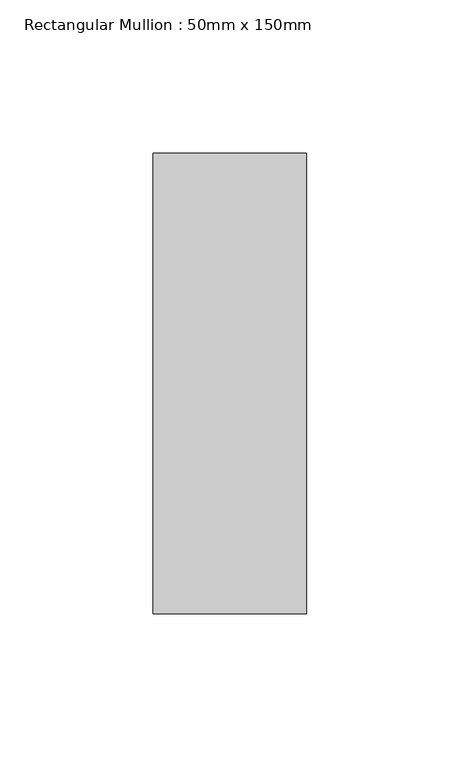
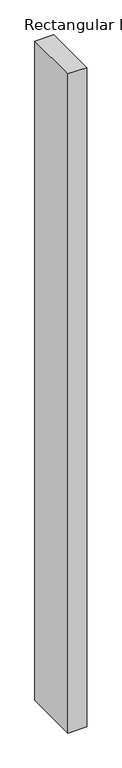
"""IFC4 building model written with IfcOpenShell, lengths in millimetres: member geometry, Rectangular Mullion : 50mm x 150mm."""

import ifcopenshell
import ifcopenshell.guid

model = None  # the IFC model being written
_history = None  # IfcOwnerHistory: only IFC2X3 demands one
_inside = {}  # id of a spatial element -> (the spatial element, [elements in it])
_under = {}  # id of a project, library or spatial element -> (it, [spatial elements below it])
_declared = {}  # id of a project -> (the project, [libraries it declares])
_typed = {}  # id of a type object -> (the type object, [elements of that type])
_made_of = {}  # id of a material, layer set ... -> (it, [elements and type objects made of it])


def new_model(schema):
    """Start an empty IFC model of exactly this schema.

    Asked for "IFC4X3", IfcOpenShell would pick the latest addendum, in which some entities
    have other attributes; the version numbers below select the first issue.
    IFC2X3 requires an IfcOwnerHistory on every rooted entity: one is made here for all.
    """
    global model, _history
    if schema == "IFC4X3":
        model = ifcopenshell.file(schema_version=(4, 3, 0, 0))
    else:
        model = ifcopenshell.file(schema=schema)
    _inside.clear()
    _under.clear()
    _declared.clear()
    _typed.clear()
    _made_of.clear()
    _history = None
    if model.schema == "IFC2X3":
        org = make("IfcOrganization", Name="unknown")
        user = make(
            "IfcPersonAndOrganization",
            ThePerson=make("IfcPerson", FamilyName="unknown"),
            TheOrganization=org,
        )
        app = make(
            "IfcApplication",
            ApplicationDeveloper=org,
            Version="unknown",
            ApplicationFullName="unknown",
            ApplicationIdentifier="unknown",
        )
        _history = make(
            "IfcOwnerHistory",
            OwningUser=user,
            OwningApplication=app,
            ChangeAction="ADDED",
            CreationDate=0,
        )
    return model


def make(cls, **values):
    """One entity of the class cls with the attributes given. An attribute that is None is left unset."""
    return model.create_entity(
        cls, **{name: value for name, value in values.items() if value is not None}
    )


def rooted(cls, **values):
    """An entity with a GlobalId (a new one), such as an element, a storey or a relation."""
    return make(cls, GlobalId=ifcopenshell.guid.new(), OwnerHistory=_history, **values)


def si_unit(unit_type, name, prefix=None):
    """IfcSIUnit, for example si_unit("LENGTHUNIT", "METRE", prefix="MILLI")."""
    return make("IfcSIUnit", UnitType=unit_type, Prefix=prefix, Name=name)


def assignment(units):
    """IfcUnitAssignment: the units of a project."""
    return None if units is None else make("IfcUnitAssignment", Units=units)


def point(xyz):
    """IfcCartesianPoint."""
    return None if xyz is None else make("IfcCartesianPoint", Coordinates=xyz)


def direction(xyz):
    """IfcDirection."""
    return None if xyz is None else make("IfcDirection", DirectionRatios=xyz)


def frame(location, z_axis=None, x_axis=None):
    """IfcAxis2Placement3D, a coordinate frame: its origin and axes. An axis left out is left unset."""
    return make(
        "IfcAxis2Placement3D",
        Location=point(location),
        Axis=direction(z_axis),
        RefDirection=direction(x_axis),
    )


def origin():
    """The frame at (0, 0, 0) with its axes left unset."""
    return frame((0.0, 0.0, 0.0))


def place(relative_to, where):
    """IfcLocalPlacement: puts the frame where relative to a parent placement (None: the world)."""
    return make(
        "IfcLocalPlacement", PlacementRelTo=relative_to, RelativePlacement=where
    )


def context(
    kind, dimensions, precision=None, world=None, true_north=None, identifier=None
):
    """IfcGeometricRepresentationContext, for example the 3D "Model" context."""
    return make(
        "IfcGeometricRepresentationContext",
        ContextIdentifier=identifier,
        ContextType=kind,
        CoordinateSpaceDimension=dimensions,
        Precision=precision,
        WorldCoordinateSystem=world,
        TrueNorth=true_north,
    )


def project(units=None, contexts=None):
    """IfcProject with its units and contexts."""
    return rooted(
        "IfcProject",
        Name="project",
        RepresentationContexts=contexts,
        UnitsInContext=assignment(units),
    )


def spatial(cls, under=None, at=None, **own):
    """A site, building, storey or space (cls), placed at a placement, below another one or the project."""
    s = rooted(cls, ObjectPlacement=at, **own)
    if under is not None:
        _under.setdefault(under.id(), (under, []))[1].append(s)
    return s


def polyline(points):
    """IfcPolyline through the points."""
    return make("IfcPolyline", Points=[point(p) for p in points])


def outline(outer, holes=None, kind="AREA"):
    """IfcArbitraryClosedProfileDef: a profile drawn as a closed curve; with holes, ...WithVoids."""
    if holes is None:
        return make("IfcArbitraryClosedProfileDef", ProfileType=kind, OuterCurve=outer)
    return make(
        "IfcArbitraryProfileDefWithVoids",
        ProfileType=kind,
        OuterCurve=outer,
        InnerCurves=holes,
    )


def extrude(swept, where, along, depth):
    """IfcExtrudedAreaSolid: the profile swept, set in the frame where, extruded along a direction by depth."""
    return make(
        "IfcExtrudedAreaSolid",
        SweptArea=swept,
        Position=where,
        ExtrudedDirection=direction(along),
        Depth=depth,
    )


def shape(context_of_items, identifier, shape_type, items):
    """IfcShapeRepresentation: the items that make up one representation, for example the "Body"."""
    return make(
        "IfcShapeRepresentation",
        ContextOfItems=context_of_items,
        RepresentationIdentifier=identifier,
        RepresentationType=shape_type,
        Items=items,
    )


def source(mapping_origin, context_of_items, identifier, shape_type, items):
    """IfcRepresentationMap: a shape defined once, which mapped items show again and again."""
    return make(
        "IfcRepresentationMap",
        MappingOrigin=mapping_origin,
        MappedRepresentation=shape(context_of_items, identifier, shape_type, items),
    )


def transform(
    local_origin,
    x_axis=None,
    y_axis=None,
    z_axis=None,
    scale=None,
    scale2=None,
    scale3=None,
    uniform=True,
):
    """IfcCartesianTransformationOperator3D, or its non-uniform kind. x_axis, y_axis, z_axis: its Axis1, 2, 3."""
    if uniform:
        return make(
            "IfcCartesianTransformationOperator3D",
            Axis1=direction(x_axis),
            Axis2=direction(y_axis),
            LocalOrigin=point(local_origin),
            Scale=scale,
            Axis3=direction(z_axis),
        )
    return make(
        "IfcCartesianTransformationOperator3DnonUniform",
        Axis1=direction(x_axis),
        Axis2=direction(y_axis),
        LocalOrigin=point(local_origin),
        Scale=scale,
        Axis3=direction(z_axis),
        Scale2=scale2,
        Scale3=scale3,
    )


def mapped(mapping_source, mapping_target):
    """IfcMappedItem: shows the shape of a source again, moved by a transform."""
    return make(
        "IfcMappedItem", MappingSource=mapping_source, MappingTarget=mapping_target
    )


def made_of(thing, what):
    """Note that an element or type object is made of a material, layer set ...; save() writes the relation."""
    if what is not None:
        _made_of.setdefault(what.id(), (what, []))[1].append(thing)
    return thing


def element(
    cls,
    number,
    at=None,
    inside=None,
    cuts=None,
    type_object=None,
    material=None,
    context=None,
    identifier="Body",
    shape_type=None,
    held_by="IfcProductDefinitionShape",
    body=None,
    shapes=None,
    **own,
):
    """One element of the class cls, such as IfcWall. Its Tag is "e" and its number.

    at: its placement. inside: the storey or other place that contains it. cuts: it is an
    opening in that element (IfcRelVoidsElement). A single representation is given by context,
    identifier, shape_type and body (its items); several are given by shapes. held_by: the class
    of the entity that holds the representations. save() writes the other relations.
    """
    e = rooted(cls, Tag="e%d" % number, ObjectPlacement=at, **own)
    if body is not None:
        shapes = [shape(context, identifier, shape_type, body)]
    if shapes is not None:
        e.Representation = make(held_by, Representations=shapes)
    if inside is not None:
        _inside.setdefault(inside.id(), (inside, []))[1].append(e)
    if cuts is not None:
        rooted(
            "IfcRelVoidsElement", RelatingBuildingElement=cuts, RelatedOpeningElement=e
        )
    if type_object is not None:
        _typed.setdefault(type_object.id(), (type_object, []))[1].append(e)
    return made_of(e, material)


def aggregate(whole, parts):
    """IfcRelAggregates: a whole, such as a stair, and the parts it consists of."""
    return rooted("IfcRelAggregates", RelatingObject=whole, RelatedObjects=parts)


def save(model, path):
    """Write the relations noted so far, then the file.

    IfcRelAggregates (storeys below a building ...), IfcRelContainedInSpatialStructure (elements
    in a storey), IfcRelDefinesByType, IfcRelAssociatesMaterial and IfcRelDeclares: one each for
    every whole, place, type object, material and project.
    """
    for whole, parts in _under.values():
        aggregate(whole, parts)
    for where, things in _inside.values():
        rooted(
            "IfcRelContainedInSpatialStructure",
            RelatedElements=things,
            RelatingStructure=where,
        )
    for kind, things in _typed.values():
        rooted("IfcRelDefinesByType", RelatedObjects=things, RelatingType=kind)
    for what, things in _made_of.values():
        rooted("IfcRelAssociatesMaterial", RelatedObjects=things, RelatingMaterial=what)
    for by, libraries in _declared.values():
        rooted("IfcRelDeclares", RelatingContext=by, RelatedDefinitions=libraries)
    model.write(path)


def rectangular_mullion_50mm_x_150mm_3e3f77b8(model_context):
    return source(origin(), model_context, "Body", "SweptSolid", [
        extrude(outline(polyline([(25.0, 75.0), (25.0, -75.0), (-25.0, -75.0), (-25.0, 75.0), (25.0, 75.0)])), frame((0.0, 0.0, -1830.0000003), z_axis=(0.0, 0.0, 1.0), x_axis=(1.0, 0.0, 0.0)), (0.0, 0.0, 1.0), 1830.0000003),
    ])


if __name__ == "__main__":
    model = new_model("IFC4")
    model_context = context("Model", 3, world=origin())
    ifc_project = project(units=[si_unit("LENGTHUNIT", "METRE", prefix="MILLI")], contexts=[model_context])
    site = spatial("IfcSite", under=ifc_project)
    building = spatial("IfcBuilding", under=site)
    placement = place(None, origin())
    rectangular_mullion_50mm_x_150mm_shape = rectangular_mullion_50mm_x_150mm_3e3f77b8(model_context)
    element("IfcMember", 1, ObjectType="Rectangular Mullion : 50mm x 150mm", at=placement, inside=building, context=model_context, shape_type="MappedRepresentation", body=[
        mapped(rectangular_mullion_50mm_x_150mm_shape, transform((0.0, 0.0, 0.0), x_axis=(1.0, 0.0, 0.0), y_axis=(0.0, 1.0, 0.0), z_axis=(0.0, 0.0, 1.0))),
    ])
    save(model, "model.ifc")

# Revit data of these elements
# Type "Rectangular Mullion : 50mm x 150mm"
#   built-in parameter 1007304 = 0.492126 (stored number, unit not read)
#   built-in parameter 1007301 = 0.082021 (stored number, unit not read)
#   built-in parameter 1007300 = 0.082021 (stored number, unit not read)
# Element 1 (IfcMember, "Rectangular Mullion : 50mm x 150mm")
#   Materials on its faces: "Aluminum"
# Materials
#   "Aluminum": class "Metal", colour RGB 244 244 244, transparency 0, Description = "Aluminum 6061", Cost = 0
